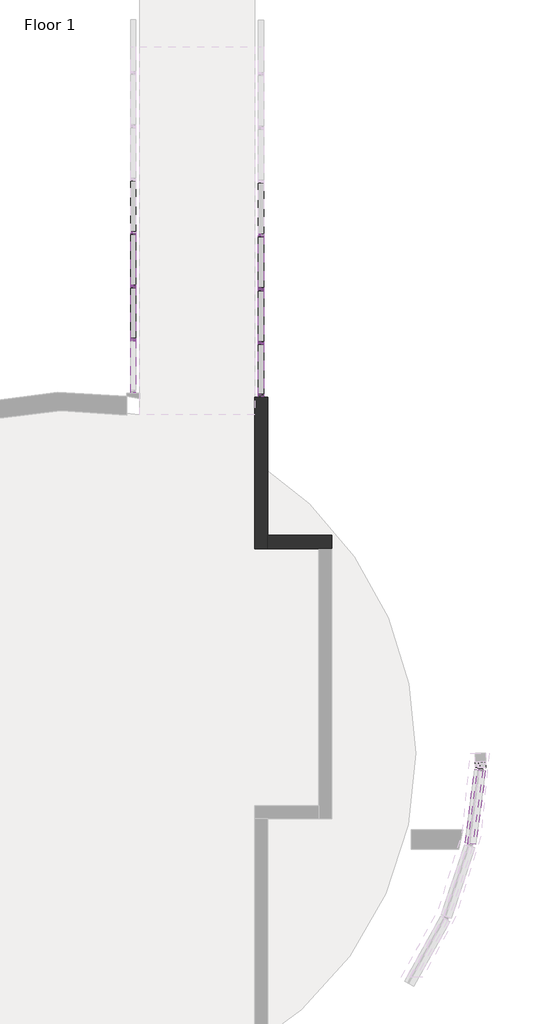
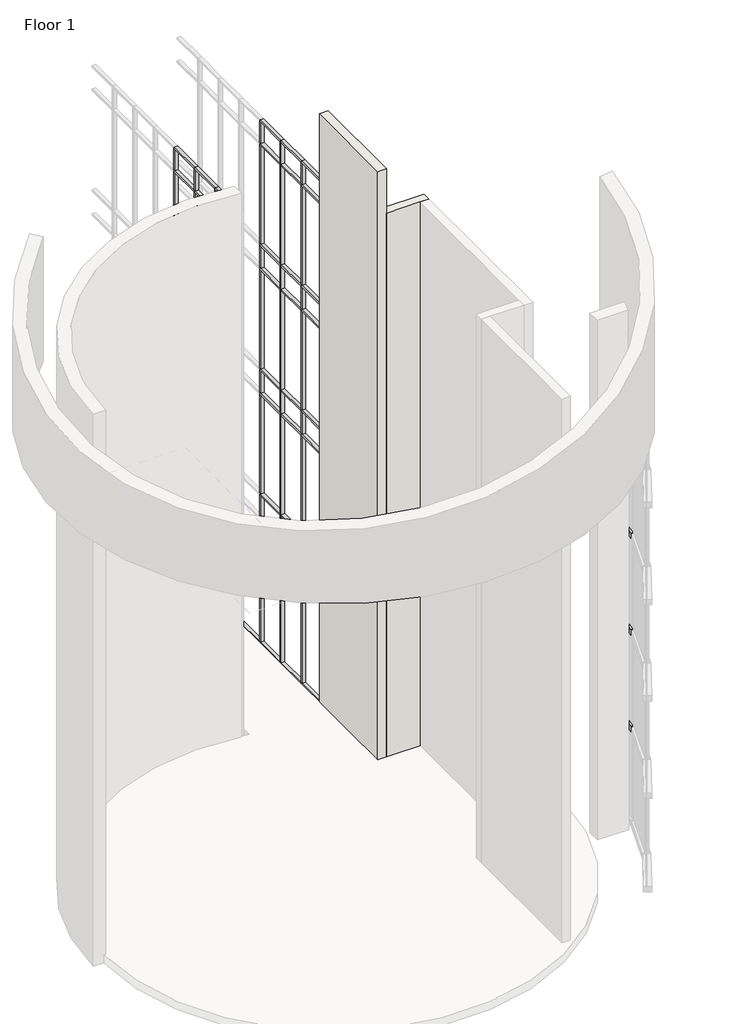
# One storey, part 7 of 11: 111 members, 2 walls.
"""IFC4 building model written with IfcOpenShell, lengths in millimetres."""

import ifcopenshell
import ifcopenshell.guid

model = None  # the IFC model being written
_history = None  # IfcOwnerHistory: only IFC2X3 demands one
_inside = {}  # id of a spatial element -> (the spatial element, [elements in it])
_under = {}  # id of a project, library or spatial element -> (it, [spatial elements below it])
_declared = {}  # id of a project -> (the project, [libraries it declares])
_typed = {}  # id of a type object -> (the type object, [elements of that type])
_made_of = {}  # id of a material, layer set ... -> (it, [elements and type objects made of it])


def new_model(schema):
    """Start an empty IFC model of exactly this schema.

    Asked for "IFC4X3", IfcOpenShell would pick the latest addendum, in which some entities
    have other attributes; the version numbers below select the first issue.
    IFC2X3 requires an IfcOwnerHistory on every rooted entity: one is made here for all.
    """
    global model, _history
    if schema == "IFC4X3":
        model = ifcopenshell.file(schema_version=(4, 3, 0, 0))
    else:
        model = ifcopenshell.file(schema=schema)
    _inside.clear()
    _under.clear()
    _declared.clear()
    _typed.clear()
    _made_of.clear()
    _history = None
    if model.schema == "IFC2X3":
        org = make("IfcOrganization", Name="unknown")
        user = make(
            "IfcPersonAndOrganization",
            ThePerson=make("IfcPerson", FamilyName="unknown"),
            TheOrganization=org,
        )
        app = make(
            "IfcApplication",
            ApplicationDeveloper=org,
            Version="unknown",
            ApplicationFullName="unknown",
            ApplicationIdentifier="unknown",
        )
        _history = make(
            "IfcOwnerHistory",
            OwningUser=user,
            OwningApplication=app,
            ChangeAction="ADDED",
            CreationDate=0,
        )
    return model


def make(cls, **values):
    """One entity of the class cls with the attributes given. An attribute that is None is left unset."""
    return model.create_entity(
        cls, **{name: value for name, value in values.items() if value is not None}
    )


def rooted(cls, **values):
    """An entity with a GlobalId (a new one), such as an element, a storey or a relation."""
    return make(cls, GlobalId=ifcopenshell.guid.new(), OwnerHistory=_history, **values)


def si_unit(unit_type, name, prefix=None):
    """IfcSIUnit, for example si_unit("LENGTHUNIT", "METRE", prefix="MILLI")."""
    return make("IfcSIUnit", UnitType=unit_type, Prefix=prefix, Name=name)


def assignment(units):
    """IfcUnitAssignment: the units of a project."""
    return None if units is None else make("IfcUnitAssignment", Units=units)


def point(xyz):
    """IfcCartesianPoint."""
    return None if xyz is None else make("IfcCartesianPoint", Coordinates=xyz)


def direction(xyz):
    """IfcDirection."""
    return None if xyz is None else make("IfcDirection", DirectionRatios=xyz)


def frame(location, z_axis=None, x_axis=None):
    """IfcAxis2Placement3D, a coordinate frame: its origin and axes. An axis left out is left unset."""
    return make(
        "IfcAxis2Placement3D",
        Location=point(location),
        Axis=direction(z_axis),
        RefDirection=direction(x_axis),
    )


def origin():
    """The frame at (0, 0, 0) with its axes left unset."""
    return frame((0.0, 0.0, 0.0))


def place(relative_to, where):
    """IfcLocalPlacement: puts the frame where relative to a parent placement (None: the world)."""
    return make(
        "IfcLocalPlacement", PlacementRelTo=relative_to, RelativePlacement=where
    )


def context(
    kind, dimensions, precision=None, world=None, true_north=None, identifier=None
):
    """IfcGeometricRepresentationContext, for example the 3D "Model" context."""
    return make(
        "IfcGeometricRepresentationContext",
        ContextIdentifier=identifier,
        ContextType=kind,
        CoordinateSpaceDimension=dimensions,
        Precision=precision,
        WorldCoordinateSystem=world,
        TrueNorth=true_north,
    )


def project(units=None, contexts=None):
    """IfcProject with its units and contexts."""
    return rooted(
        "IfcProject",
        Name="project",
        RepresentationContexts=contexts,
        UnitsInContext=assignment(units),
    )


def spatial(cls, under=None, at=None, **own):
    """A site, building, storey or space (cls), placed at a placement, below another one or the project."""
    s = rooted(cls, ObjectPlacement=at, **own)
    if under is not None:
        _under.setdefault(under.id(), (under, []))[1].append(s)
    return s


def polyline(points):
    """IfcPolyline through the points."""
    return make("IfcPolyline", Points=[point(p) for p in points])


def outline(outer, holes=None, kind="AREA"):
    """IfcArbitraryClosedProfileDef: a profile drawn as a closed curve; with holes, ...WithVoids."""
    if holes is None:
        return make("IfcArbitraryClosedProfileDef", ProfileType=kind, OuterCurve=outer)
    return make(
        "IfcArbitraryProfileDefWithVoids",
        ProfileType=kind,
        OuterCurve=outer,
        InnerCurves=holes,
    )


def extrude(swept, where, along, depth):
    """IfcExtrudedAreaSolid: the profile swept, set in the frame where, extruded along a direction by depth."""
    return make(
        "IfcExtrudedAreaSolid",
        SweptArea=swept,
        Position=where,
        ExtrudedDirection=direction(along),
        Depth=depth,
    )


def faces_of(points, faces, orient=None, outer=None):
    """IfcFace entities. A face is a list of loops; a loop is a list of indices into points, from 0.

    orient and outer hold one flag for each loop. By default every Orientation is true, the
    first loop of a face is its IfcFaceOuterBound and the others are IfcFaceBound.
    """
    made = []
    for i, loops in enumerate(faces):
        bounds = []
        for j, loop in enumerate(loops):
            is_outer = j == 0 if outer is None else outer[i][j]
            bounds.append(
                make(
                    "IfcFaceOuterBound" if is_outer else "IfcFaceBound",
                    Bound=make("IfcPolyLoop", Polygon=[points[k] for k in loop]),
                    Orientation=True if orient is None else orient[i][j],
                )
            )
        made.append(make("IfcFace", Bounds=bounds))
    return made


def faceted_brep(points, faces, orient=None, outer=None, voids=None):
    """IfcFacetedBrep: a solid bounded by flat faces; with voids (closed shells), ...WithVoids."""
    shared = [point(p) for p in points]
    hull = make("IfcClosedShell", CfsFaces=faces_of(shared, faces, orient, outer))
    if voids is None:
        return make("IfcFacetedBrep", Outer=hull)
    return make(
        "IfcFacetedBrepWithVoids",
        Outer=hull,
        Voids=[
            make(cls, CfsFaces=faces_of(shared, fs, o, b)) for cls, fs, o, b in voids
        ],
    )


def shape(context_of_items, identifier, shape_type, items):
    """IfcShapeRepresentation: the items that make up one representation, for example the "Body"."""
    return make(
        "IfcShapeRepresentation",
        ContextOfItems=context_of_items,
        RepresentationIdentifier=identifier,
        RepresentationType=shape_type,
        Items=items,
    )


def source(mapping_origin, context_of_items, identifier, shape_type, items):
    """IfcRepresentationMap: a shape defined once, which mapped items show again and again."""
    return make(
        "IfcRepresentationMap",
        MappingOrigin=mapping_origin,
        MappedRepresentation=shape(context_of_items, identifier, shape_type, items),
    )


def transform(
    local_origin,
    x_axis=None,
    y_axis=None,
    z_axis=None,
    scale=None,
    scale2=None,
    scale3=None,
    uniform=True,
):
    """IfcCartesianTransformationOperator3D, or its non-uniform kind. x_axis, y_axis, z_axis: its Axis1, 2, 3."""
    if uniform:
        return make(
            "IfcCartesianTransformationOperator3D",
            Axis1=direction(x_axis),
            Axis2=direction(y_axis),
            LocalOrigin=point(local_origin),
            Scale=scale,
            Axis3=direction(z_axis),
        )
    return make(
        "IfcCartesianTransformationOperator3DnonUniform",
        Axis1=direction(x_axis),
        Axis2=direction(y_axis),
        LocalOrigin=point(local_origin),
        Scale=scale,
        Axis3=direction(z_axis),
        Scale2=scale2,
        Scale3=scale3,
    )


def mapped(mapping_source, mapping_target):
    """IfcMappedItem: shows the shape of a source again, moved by a transform."""
    return make(
        "IfcMappedItem", MappingSource=mapping_source, MappingTarget=mapping_target
    )


def made_of(thing, what):
    """Note that an element or type object is made of a material, layer set ...; save() writes the relation."""
    if what is not None:
        _made_of.setdefault(what.id(), (what, []))[1].append(thing)
    return thing


def element(
    cls,
    number,
    at=None,
    inside=None,
    cuts=None,
    type_object=None,
    material=None,
    context=None,
    identifier="Body",
    shape_type=None,
    held_by="IfcProductDefinitionShape",
    body=None,
    shapes=None,
    **own,
):
    """One element of the class cls, such as IfcWall. Its Tag is "e" and its number.

    at: its placement. inside: the storey or other place that contains it. cuts: it is an
    opening in that element (IfcRelVoidsElement). A single representation is given by context,
    identifier, shape_type and body (its items); several are given by shapes. held_by: the class
    of the entity that holds the representations. save() writes the other relations.
    """
    e = rooted(cls, Tag="e%d" % number, ObjectPlacement=at, **own)
    if body is not None:
        shapes = [shape(context, identifier, shape_type, body)]
    if shapes is not None:
        e.Representation = make(held_by, Representations=shapes)
    if inside is not None:
        _inside.setdefault(inside.id(), (inside, []))[1].append(e)
    if cuts is not None:
        rooted(
            "IfcRelVoidsElement", RelatingBuildingElement=cuts, RelatedOpeningElement=e
        )
    if type_object is not None:
        _typed.setdefault(type_object.id(), (type_object, []))[1].append(e)
    return made_of(e, material)


def aggregate(whole, parts):
    """IfcRelAggregates: a whole, such as a stair, and the parts it consists of."""
    return rooted("IfcRelAggregates", RelatingObject=whole, RelatedObjects=parts)


def save(model, path):
    """Write the relations noted so far, then the file.

    IfcRelAggregates (storeys below a building ...), IfcRelContainedInSpatialStructure (elements
    in a storey), IfcRelDefinesByType, IfcRelAssociatesMaterial and IfcRelDeclares: one each for
    every whole, place, type object, material and project.
    """
    for whole, parts in _under.values():
        aggregate(whole, parts)
    for where, things in _inside.values():
        rooted(
            "IfcRelContainedInSpatialStructure",
            RelatedElements=things,
            RelatingStructure=where,
        )
    for kind, things in _typed.values():
        rooted("IfcRelDefinesByType", RelatedObjects=things, RelatingType=kind)
    for what, things in _made_of.values():
        rooted("IfcRelAssociatesMaterial", RelatedObjects=things, RelatingMaterial=what)
    for by, libraries in _declared.values():
        rooted("IfcRelDeclares", RelatingContext=by, RelatedDefinitions=libraries)
    model.write(path)


def member_5d07894b(model_context):
    return source(origin(), model_context, "Body", "SweptSolid", [
        extrude(outline(polyline([(31.75, 63.5), (31.75, -63.5), (-31.75, -63.5), (-31.75, 63.5), (31.75, 63.5)])), frame((0.0, 0.0, -4629.15), z_axis=(0.0, 0.0, 1.0), x_axis=(1.0, 0.0, 0.0)), (0.0, 0.0, 1.0), 4629.15),
    ])


def member_c86c7f77(model_context):
    return source(origin(), model_context, "Body", "SweptSolid", [
        extrude(outline(polyline([(31.75, 63.5), (31.75, -63.5), (-31.75, -63.5), (-31.75, 63.5), (31.75, 63.5)])), frame((0.0, 0.0, -1270.9989637), z_axis=(0.0, 0.0, 1.0), x_axis=(1.0, 0.0, 0.0)), (0.0, 0.0, 1.0), 1270.9989637),
    ])


def member_60e3aab2(model_context):
    return source(origin(), model_context, "Body", "SweptSolid", [
        extrude(outline(polyline([(0.0, 63.5), (0.0, -63.5), (-63.5, -63.5), (-63.5, 63.5), (0.0, 63.5)])), frame((0.0, 0.0, -1270.9989637), z_axis=(0.0, 0.0, 1.0), x_axis=(1.0, 0.0, 0.0)), (0.0, 0.0, 1.0), 1270.9989637),
    ])


def member_3ba9e939(model_context):
    return source(origin(), model_context, "Body", "SweptSolid", [
        extrude(outline(polyline([(31.75, 63.5), (31.75, -63.5), (-31.75, -63.5), (-31.75, 63.5), (31.75, 63.5)])), frame((0.0, 0.0, -3746.5), z_axis=(0.0, 0.0, 1.0), x_axis=(1.0, 0.0, 0.0)), (0.0, 0.0, 1.0), 3746.5),
    ])


def member_ad567e07(model_context):
    return source(origin(), model_context, "Body", "SweptSolid", [
        extrude(outline(polyline([(31.75, 63.5), (31.75, -63.5), (-31.75, -63.5), (-31.75, 63.5), (31.75, 63.5)])), frame((0.0, 0.0, -819.15), z_axis=(0.0, 0.0, 1.0), x_axis=(1.0, 0.0, 0.0)), (0.0, 0.0, 1.0), 819.15),
    ])


def member_7db1855a(model_context):
    return source(origin(), model_context, "Body", "SweptSolid", [
        extrude(outline(polyline([(31.75, 63.5), (31.75, -63.5), (-31.75, -63.5), (-31.75, 63.5), (31.75, 63.5)])), frame((0.0, 0.0, -850.9), z_axis=(0.0, 0.0, 1.0), x_axis=(1.0, 0.0, 0.0)), (0.0, 0.0, 1.0), 850.9),
    ])


def member_5783932f(model_context):
    return source(origin(), model_context, "Body", "SweptSolid", [
        extrude(outline(polyline([(0.0, 63.5), (0.0, -63.5), (-63.5, -63.5), (-63.5, 63.5), (0.0, 63.5)])), frame((0.0, 0.0, -1282.7), z_axis=(0.0, 0.0, 1.0), x_axis=(1.0, 0.0, 0.0)), (0.0, 0.0, 1.0), 1282.7),
    ])


def member_98b79ab6(model_context):
    return source(origin(), model_context, "Body", "SweptSolid", [
        extrude(outline(polyline([(31.75, 63.5), (31.75, -63.5), (-31.75, -63.5), (-31.75, 63.5), (31.75, 63.5)])), frame((0.0, 0.0, -1282.7), z_axis=(0.0, 0.0, 1.0), x_axis=(1.0, 0.0, 0.0)), (0.0, 0.0, 1.0), 1282.7),
    ])


def member_810865a4(model_context):
    return source(origin(), model_context, "Body", "SweptSolid", [
        extrude(outline(polyline([(31.75, 63.5), (31.75, -63.5), (-31.75, -63.5), (-31.75, 63.5), (31.75, 63.5)])), frame((0.0, 0.0, -3657.6), z_axis=(0.0, 0.0, 1.0), x_axis=(1.0, 0.0, 0.0)), (0.0, 0.0, 1.0), 3657.6),
    ])


def member_b9454cfc(model_context):
    return source(origin(), model_context, "Body", "SweptSolid", [
        extrude(outline(polyline([(-63.5, 28.7582862), (-60.2336356, -5.8295375), (63.5, 5.8554746), (63.5, -1771.1554746), (-60.2336356, -1759.4704625), (-63.5, -1794.0582862), (-63.5, 28.7582862)])), frame((-63.5, 0.0, 0.0), z_axis=(1.0, 0.0, 0.0), x_axis=(0.0, 1.0, 0.0)), (0.0, 0.0, 1.0), 63.5),
    ])


def member_c17f1be2(model_context):
    return source(origin(), model_context, "Body", "SweptSolid", [
        extrude(outline(polyline([(0.0, 63.5), (0.0, -63.5), (-63.5, -63.5), (-63.5, 63.5), (0.0, 63.5)])), frame((0.0, 0.0, -819.15), z_axis=(0.0, 0.0, 1.0), x_axis=(1.0, 0.0, 0.0)), (0.0, 0.0, 1.0), 819.15),
    ])


def member_d2e7e466(model_context):
    return source(origin(), model_context, "Body", "SweptSolid", [
        extrude(outline(polyline([(0.0, 63.5), (0.0, -63.5), (-63.5, -63.5), (-63.5, 63.5), (0.0, 63.5)])), frame((0.0, 0.0, -850.9), z_axis=(0.0, 0.0, 1.0), x_axis=(1.0, 0.0, 0.0)), (0.0, 0.0, 1.0), 850.9),
    ])


def member_bbf28ac8(model_context):
    return source(origin(), model_context, "Body", "SweptSolid", [
        extrude(outline(polyline([(0.0, 63.5), (0.0, -63.5), (-63.5, -63.5), (-63.5, 63.5), (0.0, 63.5)])), frame((0.0, 0.0, -3746.5), z_axis=(0.0, 0.0, 1.0), x_axis=(1.0, 0.0, 0.0)), (0.0, 0.0, 1.0), 3746.5),
    ])


def member_5c8c9790(model_context):
    return source(origin(), model_context, "Body", "SweptSolid", [
        extrude(outline(polyline([(0.0, 63.5), (0.0, -63.5), (-63.5, -63.5), (-63.5, 63.5), (0.0, 63.5)])), frame((0.0, 0.0, -4629.15), z_axis=(0.0, 0.0, 1.0), x_axis=(1.0, 0.0, 0.0)), (0.0, 0.0, 1.0), 4629.15),
    ])


def member_93925f5f(model_context):
    return source(origin(), model_context, "Body", "SweptSolid", [
        extrude(outline(polyline([(0.0, 127.0), (0.0, -127.0), (-203.2, -127.0), (-203.2, 127.0), (0.0, 127.0)])), frame((0.0, 0.0, -139.2998379), z_axis=(0.0, 0.0, 1.0), x_axis=(1.0, 0.0, 0.0)), (0.0, 0.0, 1.0), 139.2998379),
    ])


def member_707c4438(model_context):
    return source(origin(), model_context, "Body", "SweptSolid", [
        extrude(outline(polyline([(101.6, 127.0), (101.6, -127.0), (-101.6, -127.0), (-101.6, 127.0), (101.6, 127.0)])), frame((0.0, 0.0, -1765.3), z_axis=(0.0, 0.0, 1.0), x_axis=(1.0, 0.0, 0.0)), (0.0, 0.0, 1.0), 1765.3),
    ])


model = new_model("IFC4")

# Units and contexts
model_context = context("Model", 3, world=origin())
ifc_project = project(units=[si_unit("LENGTHUNIT", "METRE", prefix="MILLI")], contexts=[model_context])

# Site, building, storey
site = spatial("IfcSite", under=ifc_project)
building = spatial("IfcBuilding", under=site)
storey = spatial("IfcBuildingStorey", under=building, Name="Floor 1", Elevation=0.0)

# Members
placement = place(None, origin())
member_shape = member_5d07894b(model_context)
element("IfcMember", 1, ObjectType="Rectangular Mullion1 : 2.5\" x 5\" rectangular", at=placement, inside=storey, context=model_context, shape_type="MappedRepresentation", body=[
    mapped(member_shape, transform((10878.8276119, 30390.311889, -88.9), x_axis=(0.0, 1.0, 0.0), y_axis=(1.0, 0.0, 0.0), z_axis=(0.0, 0.0, -1.0))),
])
element("IfcMember", 2, ObjectType="Rectangular Mullion1 : 2.5\" x 5\" rectangular", at=placement, inside=storey, context=model_context, shape_type="MappedRepresentation", body=[
    mapped(member_shape, transform((10878.8276119, 29107.611889, -88.9), x_axis=(0.0, 1.0, 0.0), y_axis=(1.0, 0.0, 0.0), z_axis=(0.0, 0.0, -1.0))),
])
element("IfcMember", 3, ObjectType="Rectangular Mullion1 : 2.5\" x 5\" rectangular", at=placement, inside=storey, context=model_context, shape_type="MappedRepresentation", body=[
    mapped(member_shape, transform((10878.8276119, 31673.011889, -88.9), x_axis=(0.0, 1.0, 0.0), y_axis=(1.0, 0.0, 0.0), z_axis=(0.0, 0.0, -1.0))),
])
element("IfcMember", 4, ObjectType="Rectangular Mullion1 : 2.5\" x 5\" rectangular", at=placement, inside=storey, context=model_context, shape_type="MappedRepresentation", body=[
    mapped(member_shape, transform((7830.8276119, 30460.5181066, -88.9), x_axis=(0.0, 1.0, 0.0), y_axis=(1.0, 0.0, 0.0), z_axis=(0.0, 0.0, -1.0))),
])
element("IfcMember", 5, ObjectType="Rectangular Mullion1 : 2.5\" x 5\" rectangular", at=placement, inside=storey, context=model_context, shape_type="MappedRepresentation", body=[
    mapped(member_shape, transform((7830.8276119, 31731.5170704, -88.9), x_axis=(0.0, 1.0, 0.0), y_axis=(1.0, 0.0, 0.0), z_axis=(0.0, 0.0, -1.0))),
])
member_2_shape = member_c86c7f77(model_context)
element("IfcMember", 6, ObjectType="Rectangular Mullion1 : 2.5\" x 5\" rectangular", at=placement, inside=storey, context=model_context, shape_type="MappedRepresentation", body=[
    mapped(member_2_shape, transform((7830.8276119, 31731.5170704, 5486.4), x_axis=(0.0, 0.0, 1.0), y_axis=(1.0, 0.0, 0.0), z_axis=(0.0, 1.0, 0.0))),
])
element("IfcMember", 7, ObjectType="Rectangular Mullion1 : 2.5\" x 5\" rectangular", at=placement, inside=storey, context=model_context, shape_type="MappedRepresentation", body=[
    mapped(member_2_shape, transform((7830.8276119, 30460.5181066, 5486.4), x_axis=(0.0, 0.0, 1.0), y_axis=(1.0, 0.0, 0.0), z_axis=(0.0, 1.0, 0.0))),
])
element("IfcMember", 8, ObjectType="Rectangular Mullion1 : 2.5\" x 5\" rectangular", at=placement, inside=storey, context=model_context, shape_type="MappedRepresentation", body=[
    mapped(member_2_shape, transform((7830.8276119, 31731.5170704, 10210.8), x_axis=(0.0, 0.0, 1.0), y_axis=(1.0, 0.0, 0.0), z_axis=(0.0, 1.0, 0.0))),
])
element("IfcMember", 9, ObjectType="Rectangular Mullion1 : 2.5\" x 5\" rectangular", at=placement, inside=storey, context=model_context, shape_type="MappedRepresentation", body=[
    mapped(member_2_shape, transform((7830.8276119, 30460.5181066, 10210.8), x_axis=(0.0, 0.0, 1.0), y_axis=(1.0, 0.0, 0.0), z_axis=(0.0, 1.0, 0.0))),
])
element("IfcMember", 10, ObjectType="Rectangular Mullion1 : 2.5\" x 5\" rectangular", at=placement, inside=storey, context=model_context, shape_type="MappedRepresentation", body=[
    mapped(member_2_shape, transform((7830.8276119, 31731.5170704, 14935.2), x_axis=(0.0, 0.0, 1.0), y_axis=(1.0, 0.0, 0.0), z_axis=(0.0, 1.0, 0.0))),
])
element("IfcMember", 11, ObjectType="Rectangular Mullion1 : 2.5\" x 5\" rectangular", at=placement, inside=storey, context=model_context, shape_type="MappedRepresentation", body=[
    mapped(member_2_shape, transform((7830.8276119, 30460.5181066, 14935.2), x_axis=(0.0, 0.0, 1.0), y_axis=(1.0, 0.0, 0.0), z_axis=(0.0, 1.0, 0.0))),
])
element("IfcMember", 12, ObjectType="Rectangular Mullion1 : 2.5\" x 5\" rectangular", at=placement, inside=storey, context=model_context, shape_type="MappedRepresentation", body=[
    mapped(member_2_shape, transform((7830.8276119, 31731.5170704, 18745.2), x_axis=(0.0, 0.0, 1.0), y_axis=(1.0, 0.0, 0.0), z_axis=(0.0, 1.0, 0.0))),
])
element("IfcMember", 13, ObjectType="Rectangular Mullion1 : 2.5\" x 5\" rectangular", at=placement, inside=storey, context=model_context, shape_type="MappedRepresentation", body=[
    mapped(member_2_shape, transform((7830.8276119, 30460.5181066, 18745.2), x_axis=(0.0, 0.0, 1.0), y_axis=(1.0, 0.0, 0.0), z_axis=(0.0, 1.0, 0.0))),
])
element("IfcMember", 14, ObjectType="Rectangular Mullion1 : 2.5\" x 5\" rectangular", at=placement, inside=storey, context=model_context, shape_type="MappedRepresentation", body=[
    mapped(member_2_shape, transform((7830.8276119, 31731.5170704, 14020.8), x_axis=(0.0, 0.0, 1.0), y_axis=(1.0, 0.0, 0.0), z_axis=(0.0, 1.0, 0.0))),
])
element("IfcMember", 15, ObjectType="Rectangular Mullion1 : 2.5\" x 5\" rectangular", at=placement, inside=storey, context=model_context, shape_type="MappedRepresentation", body=[
    mapped(member_2_shape, transform((7830.8276119, 30460.5181066, 14020.8), x_axis=(0.0, 0.0, 1.0), y_axis=(1.0, 0.0, 0.0), z_axis=(0.0, 1.0, 0.0))),
])
element("IfcMember", 16, ObjectType="Rectangular Mullion1 : 2.5\" x 5\" rectangular", at=placement, inside=storey, context=model_context, shape_type="MappedRepresentation", body=[
    mapped(member_2_shape, transform((7830.8276119, 31731.5170704, 9296.4), x_axis=(0.0, 0.0, 1.0), y_axis=(1.0, 0.0, 0.0), z_axis=(0.0, 1.0, 0.0))),
])
element("IfcMember", 17, ObjectType="Rectangular Mullion1 : 2.5\" x 5\" rectangular", at=placement, inside=storey, context=model_context, shape_type="MappedRepresentation", body=[
    mapped(member_2_shape, transform((7830.8276119, 30460.5181066, 9296.4), x_axis=(0.0, 0.0, 1.0), y_axis=(1.0, 0.0, 0.0), z_axis=(0.0, 1.0, 0.0))),
])
element("IfcMember", 18, ObjectType="Rectangular Mullion1 : 2.5\" x 5\" rectangular", at=placement, inside=storey, context=model_context, shape_type="MappedRepresentation", body=[
    mapped(member_2_shape, transform((7830.8276119, 31731.5170704, 4572.0), x_axis=(0.0, 0.0, 1.0), y_axis=(1.0, 0.0, 0.0), z_axis=(0.0, 1.0, 0.0))),
])
element("IfcMember", 19, ObjectType="Rectangular Mullion1 : 2.5\" x 5\" rectangular", at=placement, inside=storey, context=model_context, shape_type="MappedRepresentation", body=[
    mapped(member_2_shape, transform((7830.8276119, 30460.5181066, 4572.0), x_axis=(0.0, 0.0, 1.0), y_axis=(1.0, 0.0, 0.0), z_axis=(0.0, 1.0, 0.0))),
])
member_3_shape = member_60e3aab2(model_context)
element("IfcMember", 20, ObjectType="Rectangular Mullion1 : 2.5\" x 5\" rectangular", at=placement, inside=storey, context=model_context, shape_type="MappedRepresentation", body=[
    mapped(member_3_shape, transform((7830.8276119, 30460.5181066, -152.4), x_axis=(0.0, 0.0, -1.0), y_axis=(1.0, 0.0, 0.0), z_axis=(0.0, -1.0, 0.0))),
])
element("IfcMember", 21, ObjectType="Rectangular Mullion1 : 2.5\" x 5\" rectangular", at=placement, inside=storey, context=model_context, shape_type="MappedRepresentation", body=[
    mapped(member_3_shape, transform((7830.8276119, 31731.5170704, -152.4), x_axis=(0.0, 0.0, -1.0), y_axis=(1.0, 0.0, 0.0), z_axis=(0.0, -1.0, 0.0))),
])
element("IfcMember", 22, ObjectType="Rectangular Mullion1 : 2.5\" x 5\" rectangular", at=placement, inside=storey, context=model_context, shape_type="MappedRepresentation", body=[
    mapped(member_3_shape, transform((7830.8276119, 29189.5191429, -152.4), x_axis=(0.0, 0.0, -1.0), y_axis=(1.0, 0.0, 0.0), z_axis=(0.0, -1.0, 0.0))),
])
element("IfcMember", 23, ObjectType="Rectangular Mullion1 : 2.5\" x 5\" rectangular", at=placement, inside=storey, context=model_context, shape_type="MappedRepresentation", body=[
    mapped(member_3_shape, transform((7830.8276119, 30460.5181066, 19659.6), x_axis=(0.0, 0.0, 1.0), y_axis=(1.0, 0.0, 0.0), z_axis=(0.0, 1.0, 0.0))),
])
element("IfcMember", 24, ObjectType="Rectangular Mullion1 : 2.5\" x 5\" rectangular", at=placement, inside=storey, context=model_context, shape_type="MappedRepresentation", body=[
    mapped(member_3_shape, transform((7830.8276119, 31731.5170704, 19659.6), x_axis=(0.0, 0.0, 1.0), y_axis=(1.0, 0.0, 0.0), z_axis=(0.0, 1.0, 0.0))),
])
element("IfcMember", 25, ObjectType="Rectangular Mullion1 : 2.5\" x 5\" rectangular", at=placement, inside=storey, context=model_context, shape_type="MappedRepresentation", body=[
    mapped(member_3_shape, transform((7830.8276119, 29189.5191429, 19659.6), x_axis=(0.0, 0.0, 1.0), y_axis=(1.0, 0.0, 0.0), z_axis=(0.0, 1.0, 0.0))),
])
member_4_shape = member_3ba9e939(model_context)
element("IfcMember", 26, ObjectType="Rectangular Mullion1 : 2.5\" x 5\" rectangular", at=placement, inside=storey, context=model_context, shape_type="MappedRepresentation", body=[
    mapped(member_4_shape, transform((10878.8276119, 30390.311889, 14966.95), x_axis=(0.0, 1.0, 0.0), y_axis=(1.0, 0.0, 0.0), z_axis=(0.0, 0.0, -1.0))),
])
element("IfcMember", 27, ObjectType="Rectangular Mullion1 : 2.5\" x 5\" rectangular", at=placement, inside=storey, context=model_context, shape_type="MappedRepresentation", body=[
    mapped(member_4_shape, transform((10878.8276119, 30390.311889, 10242.55), x_axis=(0.0, 1.0, 0.0), y_axis=(1.0, 0.0, 0.0), z_axis=(0.0, 0.0, -1.0))),
])
element("IfcMember", 28, ObjectType="Rectangular Mullion1 : 2.5\" x 5\" rectangular", at=placement, inside=storey, context=model_context, shape_type="MappedRepresentation", body=[
    mapped(member_4_shape, transform((10878.8276119, 30390.311889, 5518.15), x_axis=(0.0, 1.0, 0.0), y_axis=(1.0, 0.0, 0.0), z_axis=(0.0, 0.0, -1.0))),
])
element("IfcMember", 29, ObjectType="Rectangular Mullion1 : 2.5\" x 5\" rectangular", at=placement, inside=storey, context=model_context, shape_type="MappedRepresentation", body=[
    mapped(member_4_shape, transform((10878.8276119, 29107.611889, 14966.95), x_axis=(0.0, 1.0, 0.0), y_axis=(1.0, 0.0, 0.0), z_axis=(0.0, 0.0, -1.0))),
])
element("IfcMember", 30, ObjectType="Rectangular Mullion1 : 2.5\" x 5\" rectangular", at=placement, inside=storey, context=model_context, shape_type="MappedRepresentation", body=[
    mapped(member_4_shape, transform((10878.8276119, 29107.611889, 10242.55), x_axis=(0.0, 1.0, 0.0), y_axis=(1.0, 0.0, 0.0), z_axis=(0.0, 0.0, -1.0))),
])
element("IfcMember", 31, ObjectType="Rectangular Mullion1 : 2.5\" x 5\" rectangular", at=placement, inside=storey, context=model_context, shape_type="MappedRepresentation", body=[
    mapped(member_4_shape, transform((10878.8276119, 29107.611889, 5518.15), x_axis=(0.0, 1.0, 0.0), y_axis=(1.0, 0.0, 0.0), z_axis=(0.0, 0.0, -1.0))),
])
element("IfcMember", 32, ObjectType="Rectangular Mullion1 : 2.5\" x 5\" rectangular", at=placement, inside=storey, context=model_context, shape_type="MappedRepresentation", body=[
    mapped(member_4_shape, transform((10878.8276119, 31673.011889, 14966.95), x_axis=(0.0, 1.0, 0.0), y_axis=(1.0, 0.0, 0.0), z_axis=(0.0, 0.0, -1.0))),
])
element("IfcMember", 33, ObjectType="Rectangular Mullion1 : 2.5\" x 5\" rectangular", at=placement, inside=storey, context=model_context, shape_type="MappedRepresentation", body=[
    mapped(member_4_shape, transform((10878.8276119, 31673.011889, 10242.55), x_axis=(0.0, 1.0, 0.0), y_axis=(1.0, 0.0, 0.0), z_axis=(0.0, 0.0, -1.0))),
])
element("IfcMember", 34, ObjectType="Rectangular Mullion1 : 2.5\" x 5\" rectangular", at=placement, inside=storey, context=model_context, shape_type="MappedRepresentation", body=[
    mapped(member_4_shape, transform((10878.8276119, 31673.011889, 5518.15), x_axis=(0.0, 1.0, 0.0), y_axis=(1.0, 0.0, 0.0), z_axis=(0.0, 0.0, -1.0))),
])
element("IfcMember", 35, ObjectType="Rectangular Mullion1 : 2.5\" x 5\" rectangular", at=placement, inside=storey, context=model_context, shape_type="MappedRepresentation", body=[
    mapped(member_4_shape, transform((7830.8276119, 30460.5181066, 5518.15), x_axis=(0.0, 1.0, 0.0), y_axis=(1.0, 0.0, 0.0), z_axis=(0.0, 0.0, -1.0))),
])
element("IfcMember", 36, ObjectType="Rectangular Mullion1 : 2.5\" x 5\" rectangular", at=placement, inside=storey, context=model_context, shape_type="MappedRepresentation", body=[
    mapped(member_4_shape, transform((7830.8276119, 30460.5181066, 10242.55), x_axis=(0.0, 1.0, 0.0), y_axis=(1.0, 0.0, 0.0), z_axis=(0.0, 0.0, -1.0))),
])
element("IfcMember", 37, ObjectType="Rectangular Mullion1 : 2.5\" x 5\" rectangular", at=placement, inside=storey, context=model_context, shape_type="MappedRepresentation", body=[
    mapped(member_4_shape, transform((7830.8276119, 30460.5181066, 14966.95), x_axis=(0.0, 1.0, 0.0), y_axis=(1.0, 0.0, 0.0), z_axis=(0.0, 0.0, -1.0))),
])
element("IfcMember", 38, ObjectType="Rectangular Mullion1 : 2.5\" x 5\" rectangular", at=placement, inside=storey, context=model_context, shape_type="MappedRepresentation", body=[
    mapped(member_4_shape, transform((7830.8276119, 31731.5170704, 5518.15), x_axis=(0.0, 1.0, 0.0), y_axis=(1.0, 0.0, 0.0), z_axis=(0.0, 0.0, -1.0))),
])
element("IfcMember", 39, ObjectType="Rectangular Mullion1 : 2.5\" x 5\" rectangular", at=placement, inside=storey, context=model_context, shape_type="MappedRepresentation", body=[
    mapped(member_4_shape, transform((7830.8276119, 31731.5170704, 10242.55), x_axis=(0.0, 1.0, 0.0), y_axis=(1.0, 0.0, 0.0), z_axis=(0.0, 0.0, -1.0))),
])
element("IfcMember", 40, ObjectType="Rectangular Mullion1 : 2.5\" x 5\" rectangular", at=placement, inside=storey, context=model_context, shape_type="MappedRepresentation", body=[
    mapped(member_4_shape, transform((7830.8276119, 31731.5170704, 14966.95), x_axis=(0.0, 1.0, 0.0), y_axis=(1.0, 0.0, 0.0), z_axis=(0.0, 0.0, -1.0))),
])
element("IfcMember", 41, ObjectType="Rectangular Mullion1 : 2.5\" x 5\" rectangular", at=placement, inside=storey, context=model_context, shape_type="MappedRepresentation", body=[
    mapped(member_4_shape, transform((7830.8276119, 29189.5191429, 5518.15), x_axis=(0.0, 1.0, 0.0), y_axis=(1.0, 0.0, 0.0), z_axis=(0.0, 0.0, -1.0))),
])
element("IfcMember", 42, ObjectType="Rectangular Mullion1 : 2.5\" x 5\" rectangular", at=placement, inside=storey, context=model_context, shape_type="MappedRepresentation", body=[
    mapped(member_4_shape, transform((7830.8276119, 29189.5191429, 10242.55), x_axis=(0.0, 1.0, 0.0), y_axis=(1.0, 0.0, 0.0), z_axis=(0.0, 0.0, -1.0))),
])
element("IfcMember", 43, ObjectType="Rectangular Mullion1 : 2.5\" x 5\" rectangular", at=placement, inside=storey, context=model_context, shape_type="MappedRepresentation", body=[
    mapped(member_4_shape, transform((7830.8276119, 29189.5191429, 14966.95), x_axis=(0.0, 1.0, 0.0), y_axis=(1.0, 0.0, 0.0), z_axis=(0.0, 0.0, -1.0))),
])
member_5_shape = member_ad567e07(model_context)
element("IfcMember", 44, ObjectType="Rectangular Mullion1 : 2.5\" x 5\" rectangular", at=placement, inside=storey, context=model_context, shape_type="MappedRepresentation", body=[
    mapped(member_5_shape, transform((10878.8276119, 30390.311889, 18776.95), x_axis=(0.0, 1.0, 0.0), y_axis=(1.0, 0.0, 0.0), z_axis=(0.0, 0.0, -1.0))),
])
element("IfcMember", 45, ObjectType="Rectangular Mullion1 : 2.5\" x 5\" rectangular", at=placement, inside=storey, context=model_context, shape_type="MappedRepresentation", body=[
    mapped(member_5_shape, transform((10878.8276119, 29107.611889, 18776.95), x_axis=(0.0, 1.0, 0.0), y_axis=(1.0, 0.0, 0.0), z_axis=(0.0, 0.0, -1.0))),
])
element("IfcMember", 46, ObjectType="Rectangular Mullion1 : 2.5\" x 5\" rectangular", at=placement, inside=storey, context=model_context, shape_type="MappedRepresentation", body=[
    mapped(member_5_shape, transform((10878.8276119, 31673.011889, 18776.95), x_axis=(0.0, 1.0, 0.0), y_axis=(1.0, 0.0, 0.0), z_axis=(0.0, 0.0, -1.0))),
])
element("IfcMember", 47, ObjectType="Rectangular Mullion1 : 2.5\" x 5\" rectangular", at=placement, inside=storey, context=model_context, shape_type="MappedRepresentation", body=[
    mapped(member_5_shape, transform((7830.8276119, 30460.5181066, 18776.95), x_axis=(0.0, 1.0, 0.0), y_axis=(1.0, 0.0, 0.0), z_axis=(0.0, 0.0, -1.0))),
])
element("IfcMember", 48, ObjectType="Rectangular Mullion1 : 2.5\" x 5\" rectangular", at=placement, inside=storey, context=model_context, shape_type="MappedRepresentation", body=[
    mapped(member_5_shape, transform((7830.8276119, 31731.5170704, 18776.95), x_axis=(0.0, 1.0, 0.0), y_axis=(1.0, 0.0, 0.0), z_axis=(0.0, 0.0, -1.0))),
])
element("IfcMember", 49, ObjectType="Rectangular Mullion1 : 2.5\" x 5\" rectangular", at=placement, inside=storey, context=model_context, shape_type="MappedRepresentation", body=[
    mapped(member_5_shape, transform((7830.8276119, 29189.5191429, 18776.95), x_axis=(0.0, 1.0, 0.0), y_axis=(1.0, 0.0, 0.0), z_axis=(0.0, 0.0, -1.0))),
])
member_6_shape = member_7db1855a(model_context)
element("IfcMember", 50, ObjectType="Rectangular Mullion1 : 2.5\" x 5\" rectangular", at=placement, inside=storey, context=model_context, shape_type="MappedRepresentation", body=[
    mapped(member_6_shape, transform((10878.8276119, 30390.311889, 9328.15), x_axis=(0.0, 1.0, 0.0), y_axis=(1.0, 0.0, 0.0), z_axis=(0.0, 0.0, -1.0))),
])
element("IfcMember", 51, ObjectType="Rectangular Mullion1 : 2.5\" x 5\" rectangular", at=placement, inside=storey, context=model_context, shape_type="MappedRepresentation", body=[
    mapped(member_6_shape, transform((10878.8276119, 30390.311889, 4603.75), x_axis=(0.0, 1.0, 0.0), y_axis=(1.0, 0.0, 0.0), z_axis=(0.0, 0.0, -1.0))),
])
element("IfcMember", 52, ObjectType="Rectangular Mullion1 : 2.5\" x 5\" rectangular", at=placement, inside=storey, context=model_context, shape_type="MappedRepresentation", body=[
    mapped(member_6_shape, transform((10878.8276119, 30390.311889, 14052.55), x_axis=(0.0, 1.0, 0.0), y_axis=(1.0, 0.0, 0.0), z_axis=(0.0, 0.0, -1.0))),
])
element("IfcMember", 53, ObjectType="Rectangular Mullion1 : 2.5\" x 5\" rectangular", at=placement, inside=storey, context=model_context, shape_type="MappedRepresentation", body=[
    mapped(member_6_shape, transform((10878.8276119, 29107.611889, 9328.15), x_axis=(0.0, 1.0, 0.0), y_axis=(1.0, 0.0, 0.0), z_axis=(0.0, 0.0, -1.0))),
])
element("IfcMember", 54, ObjectType="Rectangular Mullion1 : 2.5\" x 5\" rectangular", at=placement, inside=storey, context=model_context, shape_type="MappedRepresentation", body=[
    mapped(member_6_shape, transform((10878.8276119, 29107.611889, 4603.75), x_axis=(0.0, 1.0, 0.0), y_axis=(1.0, 0.0, 0.0), z_axis=(0.0, 0.0, -1.0))),
])
element("IfcMember", 55, ObjectType="Rectangular Mullion1 : 2.5\" x 5\" rectangular", at=placement, inside=storey, context=model_context, shape_type="MappedRepresentation", body=[
    mapped(member_6_shape, transform((10878.8276119, 29107.611889, 14052.55), x_axis=(0.0, 1.0, 0.0), y_axis=(1.0, 0.0, 0.0), z_axis=(0.0, 0.0, -1.0))),
])
element("IfcMember", 56, ObjectType="Rectangular Mullion1 : 2.5\" x 5\" rectangular", at=placement, inside=storey, context=model_context, shape_type="MappedRepresentation", body=[
    mapped(member_6_shape, transform((10878.8276119, 31673.011889, 9328.15), x_axis=(0.0, 1.0, 0.0), y_axis=(1.0, 0.0, 0.0), z_axis=(0.0, 0.0, -1.0))),
])
element("IfcMember", 57, ObjectType="Rectangular Mullion1 : 2.5\" x 5\" rectangular", at=placement, inside=storey, context=model_context, shape_type="MappedRepresentation", body=[
    mapped(member_6_shape, transform((10878.8276119, 31673.011889, 4603.75), x_axis=(0.0, 1.0, 0.0), y_axis=(1.0, 0.0, 0.0), z_axis=(0.0, 0.0, -1.0))),
])
element("IfcMember", 58, ObjectType="Rectangular Mullion1 : 2.5\" x 5\" rectangular", at=placement, inside=storey, context=model_context, shape_type="MappedRepresentation", body=[
    mapped(member_6_shape, transform((10878.8276119, 31673.011889, 14052.55), x_axis=(0.0, 1.0, 0.0), y_axis=(1.0, 0.0, 0.0), z_axis=(0.0, 0.0, -1.0))),
])
element("IfcMember", 59, ObjectType="Rectangular Mullion1 : 2.5\" x 5\" rectangular", at=placement, inside=storey, context=model_context, shape_type="MappedRepresentation", body=[
    mapped(member_6_shape, transform((7830.8276119, 30460.5181066, 14052.55), x_axis=(0.0, 1.0, 0.0), y_axis=(1.0, 0.0, 0.0), z_axis=(0.0, 0.0, -1.0))),
])
element("IfcMember", 60, ObjectType="Rectangular Mullion1 : 2.5\" x 5\" rectangular", at=placement, inside=storey, context=model_context, shape_type="MappedRepresentation", body=[
    mapped(member_6_shape, transform((7830.8276119, 30460.5181066, 9328.15), x_axis=(0.0, 1.0, 0.0), y_axis=(1.0, 0.0, 0.0), z_axis=(0.0, 0.0, -1.0))),
])
element("IfcMember", 61, ObjectType="Rectangular Mullion1 : 2.5\" x 5\" rectangular", at=placement, inside=storey, context=model_context, shape_type="MappedRepresentation", body=[
    mapped(member_6_shape, transform((7830.8276119, 30460.5181066, 4603.75), x_axis=(0.0, 1.0, 0.0), y_axis=(1.0, 0.0, 0.0), z_axis=(0.0, 0.0, -1.0))),
])
element("IfcMember", 62, ObjectType="Rectangular Mullion1 : 2.5\" x 5\" rectangular", at=placement, inside=storey, context=model_context, shape_type="MappedRepresentation", body=[
    mapped(member_6_shape, transform((7830.8276119, 31731.5170704, 14052.55), x_axis=(0.0, 1.0, 0.0), y_axis=(1.0, 0.0, 0.0), z_axis=(0.0, 0.0, -1.0))),
])
element("IfcMember", 63, ObjectType="Rectangular Mullion1 : 2.5\" x 5\" rectangular", at=placement, inside=storey, context=model_context, shape_type="MappedRepresentation", body=[
    mapped(member_6_shape, transform((7830.8276119, 31731.5170704, 9328.15), x_axis=(0.0, 1.0, 0.0), y_axis=(1.0, 0.0, 0.0), z_axis=(0.0, 0.0, -1.0))),
])
element("IfcMember", 64, ObjectType="Rectangular Mullion1 : 2.5\" x 5\" rectangular", at=placement, inside=storey, context=model_context, shape_type="MappedRepresentation", body=[
    mapped(member_6_shape, transform((7830.8276119, 31731.5170704, 4603.75), x_axis=(0.0, 1.0, 0.0), y_axis=(1.0, 0.0, 0.0), z_axis=(0.0, 0.0, -1.0))),
])
element("IfcMember", 65, ObjectType="Rectangular Mullion1 : 2.5\" x 5\" rectangular", at=placement, inside=storey, context=model_context, shape_type="MappedRepresentation", body=[
    mapped(member_6_shape, transform((7830.8276119, 29189.5191429, 14052.55), x_axis=(0.0, 1.0, 0.0), y_axis=(1.0, 0.0, 0.0), z_axis=(0.0, 0.0, -1.0))),
])
element("IfcMember", 66, ObjectType="Rectangular Mullion1 : 2.5\" x 5\" rectangular", at=placement, inside=storey, context=model_context, shape_type="MappedRepresentation", body=[
    mapped(member_6_shape, transform((7830.8276119, 29189.5191429, 9328.15), x_axis=(0.0, 1.0, 0.0), y_axis=(1.0, 0.0, 0.0), z_axis=(0.0, 0.0, -1.0))),
])
element("IfcMember", 67, ObjectType="Rectangular Mullion1 : 2.5\" x 5\" rectangular", at=placement, inside=storey, context=model_context, shape_type="MappedRepresentation", body=[
    mapped(member_6_shape, transform((7830.8276119, 29189.5191429, 4603.75), x_axis=(0.0, 1.0, 0.0), y_axis=(1.0, 0.0, 0.0), z_axis=(0.0, 0.0, -1.0))),
])
member_7_shape = member_5783932f(model_context)
element("IfcMember", 68, ObjectType="Rectangular Mullion1 : 2.5\" x 5\" rectangular", at=placement, inside=storey, context=model_context, shape_type="MappedRepresentation", body=[
    mapped(member_7_shape, transform((10878.8276119, 27824.911889, -152.4), x_axis=(0.0, 0.0, -1.0), y_axis=(1.0, 0.0, 0.0), z_axis=(0.0, -1.0, 0.0))),
])
member_8_shape = member_98b79ab6(model_context)
element("IfcMember", 69, ObjectType="Rectangular Mullion1 : 2.5\" x 5\" rectangular", at=placement, inside=storey, context=model_context, shape_type="MappedRepresentation", body=[
    mapped(member_8_shape, transform((10878.8276119, 29107.611889, 14935.2), x_axis=(0.0, 0.0, 1.0), y_axis=(1.0, 0.0, 0.0), z_axis=(0.0, 1.0, 0.0))),
])
element("IfcMember", 70, ObjectType="Rectangular Mullion1 : 2.5\" x 5\" rectangular", at=placement, inside=storey, context=model_context, shape_type="MappedRepresentation", body=[
    mapped(member_8_shape, transform((10878.8276119, 29107.611889, 10210.8), x_axis=(0.0, 0.0, 1.0), y_axis=(1.0, 0.0, 0.0), z_axis=(0.0, 1.0, 0.0))),
])
element("IfcMember", 71, ObjectType="Rectangular Mullion1 : 2.5\" x 5\" rectangular", at=placement, inside=storey, context=model_context, shape_type="MappedRepresentation", body=[
    mapped(member_8_shape, transform((10878.8276119, 29107.611889, 5486.4), x_axis=(0.0, 0.0, 1.0), y_axis=(1.0, 0.0, 0.0), z_axis=(0.0, 1.0, 0.0))),
])
element("IfcMember", 72, ObjectType="Rectangular Mullion1 : 2.5\" x 5\" rectangular", at=placement, inside=storey, context=model_context, shape_type="MappedRepresentation", body=[
    mapped(member_8_shape, transform((10878.8276119, 29107.611889, 9296.4), x_axis=(0.0, 0.0, 1.0), y_axis=(1.0, 0.0, 0.0), z_axis=(0.0, 1.0, 0.0))),
])
element("IfcMember", 73, ObjectType="Rectangular Mullion1 : 2.5\" x 5\" rectangular", at=placement, inside=storey, context=model_context, shape_type="MappedRepresentation", body=[
    mapped(member_8_shape, transform((10878.8276119, 29107.611889, 4572.0), x_axis=(0.0, 0.0, 1.0), y_axis=(1.0, 0.0, 0.0), z_axis=(0.0, 1.0, 0.0))),
])
element("IfcMember", 74, ObjectType="Rectangular Mullion1 : 2.5\" x 5\" rectangular", at=placement, inside=storey, context=model_context, shape_type="MappedRepresentation", body=[
    mapped(member_8_shape, transform((10878.8276119, 29107.611889, 14020.8), x_axis=(0.0, 0.0, 1.0), y_axis=(1.0, 0.0, 0.0), z_axis=(0.0, 1.0, 0.0))),
])
element("IfcMember", 75, ObjectType="Rectangular Mullion1 : 2.5\" x 5\" rectangular", at=placement, inside=storey, context=model_context, shape_type="MappedRepresentation", body=[
    mapped(member_8_shape, transform((10878.8276119, 29107.611889, 18745.2), x_axis=(0.0, 0.0, 1.0), y_axis=(1.0, 0.0, 0.0), z_axis=(0.0, 1.0, 0.0))),
])
element("IfcMember", 76, ObjectType="Rectangular Mullion1 : 2.5\" x 5\" rectangular", at=placement, inside=storey, context=model_context, shape_type="MappedRepresentation", body=[
    mapped(member_8_shape, transform((10878.8276119, 31673.011889, 14935.2), x_axis=(0.0, 0.0, 1.0), y_axis=(1.0, 0.0, 0.0), z_axis=(0.0, 1.0, 0.0))),
])
element("IfcMember", 77, ObjectType="Rectangular Mullion1 : 2.5\" x 5\" rectangular", at=placement, inside=storey, context=model_context, shape_type="MappedRepresentation", body=[
    mapped(member_8_shape, transform((10878.8276119, 30390.311889, 14935.2), x_axis=(0.0, 0.0, 1.0), y_axis=(1.0, 0.0, 0.0), z_axis=(0.0, 1.0, 0.0))),
])
element("IfcMember", 78, ObjectType="Rectangular Mullion1 : 2.5\" x 5\" rectangular", at=placement, inside=storey, context=model_context, shape_type="MappedRepresentation", body=[
    mapped(member_8_shape, transform((10878.8276119, 31673.011889, 10210.8), x_axis=(0.0, 0.0, 1.0), y_axis=(1.0, 0.0, 0.0), z_axis=(0.0, 1.0, 0.0))),
])
element("IfcMember", 79, ObjectType="Rectangular Mullion1 : 2.5\" x 5\" rectangular", at=placement, inside=storey, context=model_context, shape_type="MappedRepresentation", body=[
    mapped(member_8_shape, transform((10878.8276119, 30390.311889, 10210.8), x_axis=(0.0, 0.0, 1.0), y_axis=(1.0, 0.0, 0.0), z_axis=(0.0, 1.0, 0.0))),
])
element("IfcMember", 80, ObjectType="Rectangular Mullion1 : 2.5\" x 5\" rectangular", at=placement, inside=storey, context=model_context, shape_type="MappedRepresentation", body=[
    mapped(member_8_shape, transform((10878.8276119, 31673.011889, 5486.4), x_axis=(0.0, 0.0, 1.0), y_axis=(1.0, 0.0, 0.0), z_axis=(0.0, 1.0, 0.0))),
])
element("IfcMember", 81, ObjectType="Rectangular Mullion1 : 2.5\" x 5\" rectangular", at=placement, inside=storey, context=model_context, shape_type="MappedRepresentation", body=[
    mapped(member_8_shape, transform((10878.8276119, 30390.311889, 5486.4), x_axis=(0.0, 0.0, 1.0), y_axis=(1.0, 0.0, 0.0), z_axis=(0.0, 1.0, 0.0))),
])
element("IfcMember", 82, ObjectType="Rectangular Mullion1 : 2.5\" x 5\" rectangular", at=placement, inside=storey, context=model_context, shape_type="MappedRepresentation", body=[
    mapped(member_8_shape, transform((10878.8276119, 31673.011889, 9296.4), x_axis=(0.0, 0.0, 1.0), y_axis=(1.0, 0.0, 0.0), z_axis=(0.0, 1.0, 0.0))),
])
element("IfcMember", 83, ObjectType="Rectangular Mullion1 : 2.5\" x 5\" rectangular", at=placement, inside=storey, context=model_context, shape_type="MappedRepresentation", body=[
    mapped(member_8_shape, transform((10878.8276119, 30390.311889, 9296.4), x_axis=(0.0, 0.0, 1.0), y_axis=(1.0, 0.0, 0.0), z_axis=(0.0, 1.0, 0.0))),
])
element("IfcMember", 84, ObjectType="Rectangular Mullion1 : 2.5\" x 5\" rectangular", at=placement, inside=storey, context=model_context, shape_type="MappedRepresentation", body=[
    mapped(member_8_shape, transform((10878.8276119, 31673.011889, 4572.0), x_axis=(0.0, 0.0, 1.0), y_axis=(1.0, 0.0, 0.0), z_axis=(0.0, 1.0, 0.0))),
])
element("IfcMember", 85, ObjectType="Rectangular Mullion1 : 2.5\" x 5\" rectangular", at=placement, inside=storey, context=model_context, shape_type="MappedRepresentation", body=[
    mapped(member_8_shape, transform((10878.8276119, 30390.311889, 4572.0), x_axis=(0.0, 0.0, 1.0), y_axis=(1.0, 0.0, 0.0), z_axis=(0.0, 1.0, 0.0))),
])
element("IfcMember", 86, ObjectType="Rectangular Mullion1 : 2.5\" x 5\" rectangular", at=placement, inside=storey, context=model_context, shape_type="MappedRepresentation", body=[
    mapped(member_8_shape, transform((10878.8276119, 31673.011889, 14020.8), x_axis=(0.0, 0.0, 1.0), y_axis=(1.0, 0.0, 0.0), z_axis=(0.0, 1.0, 0.0))),
])
element("IfcMember", 87, ObjectType="Rectangular Mullion1 : 2.5\" x 5\" rectangular", at=placement, inside=storey, context=model_context, shape_type="MappedRepresentation", body=[
    mapped(member_8_shape, transform((10878.8276119, 30390.311889, 14020.8), x_axis=(0.0, 0.0, 1.0), y_axis=(1.0, 0.0, 0.0), z_axis=(0.0, 1.0, 0.0))),
])
element("IfcMember", 88, ObjectType="Rectangular Mullion1 : 2.5\" x 5\" rectangular", at=placement, inside=storey, context=model_context, shape_type="MappedRepresentation", body=[
    mapped(member_8_shape, transform((10878.8276119, 31673.011889, 18745.2), x_axis=(0.0, 0.0, 1.0), y_axis=(1.0, 0.0, 0.0), z_axis=(0.0, 1.0, 0.0))),
])
element("IfcMember", 89, ObjectType="Rectangular Mullion1 : 2.5\" x 5\" rectangular", at=placement, inside=storey, context=model_context, shape_type="MappedRepresentation", body=[
    mapped(member_8_shape, transform((10878.8276119, 30390.311889, 18745.2), x_axis=(0.0, 0.0, 1.0), y_axis=(1.0, 0.0, 0.0), z_axis=(0.0, 1.0, 0.0))),
])
element("IfcMember", 90, ObjectType="Rectangular Mullion1 : 2.5\" x 5\" rectangular", at=placement, inside=storey, context=model_context, shape_type="MappedRepresentation", body=[
    mapped(member_7_shape, transform((10878.8276119, 30390.311889, -152.4), x_axis=(0.0, 0.0, -1.0), y_axis=(1.0, 0.0, 0.0), z_axis=(0.0, -1.0, 0.0))),
])
element("IfcMember", 91, ObjectType="Rectangular Mullion1 : 2.5\" x 5\" rectangular", at=placement, inside=storey, context=model_context, shape_type="MappedRepresentation", body=[
    mapped(member_7_shape, transform((10878.8276119, 29107.611889, -152.4), x_axis=(0.0, 0.0, -1.0), y_axis=(1.0, 0.0, 0.0), z_axis=(0.0, -1.0, 0.0))),
])
element("IfcMember", 92, ObjectType="Rectangular Mullion1 : 2.5\" x 5\" rectangular", at=placement, inside=storey, context=model_context, shape_type="MappedRepresentation", body=[
    mapped(member_7_shape, transform((10878.8276119, 31673.011889, -152.4), x_axis=(0.0, 0.0, -1.0), y_axis=(1.0, 0.0, 0.0), z_axis=(0.0, -1.0, 0.0))),
])
element("IfcMember", 93, ObjectType="Rectangular Mullion1 : 2.5\" x 5\" rectangular", at=placement, inside=storey, context=model_context, shape_type="MappedRepresentation", body=[
    mapped(member_7_shape, transform((10878.8276119, 30390.311889, 19659.6), x_axis=(0.0, 0.0, 1.0), y_axis=(1.0, 0.0, 0.0), z_axis=(0.0, 1.0, 0.0))),
])
element("IfcMember", 94, ObjectType="Rectangular Mullion1 : 2.5\" x 5\" rectangular", at=placement, inside=storey, context=model_context, shape_type="MappedRepresentation", body=[
    mapped(member_7_shape, transform((10878.8276119, 31673.011889, 19659.6), x_axis=(0.0, 0.0, 1.0), y_axis=(1.0, 0.0, 0.0), z_axis=(0.0, 1.0, 0.0))),
])
element("IfcMember", 95, ObjectType="Rectangular Mullion1 : 2.5\" x 5\" rectangular", at=placement, inside=storey, context=model_context, shape_type="MappedRepresentation", body=[
    mapped(member_7_shape, transform((10878.8276119, 29107.611889, 19659.6), x_axis=(0.0, 0.0, 1.0), y_axis=(1.0, 0.0, 0.0), z_axis=(0.0, 1.0, 0.0))),
])
member_9_shape = member_810865a4(model_context)
element("IfcMember", 96, ObjectType="Rectangular Mullion1 : 2.5\" x 5\" rectangular", at=placement, inside=storey, context=model_context, shape_type="MappedRepresentation", body=[
    mapped(member_9_shape, transform((16100.9680149, 18967.1313281, 0.0), x_axis=(0.03847320751912483, 0.9992596320792662, 0.0), y_axis=(0.9992596320792662, -0.03847320751912483, 0.0), z_axis=(0.0, 0.0, -1.0))),
])
member_10_shape = member_b9454cfc(model_context)
element("IfcMember", 97, ObjectType="Rectangular Mullion1 : 2.5\" x 5\" rectangular", at=placement, inside=storey, context=model_context, shape_type="MappedRepresentation", body=[
    mapped(member_10_shape, transform((16096.7690235, 18935.6602148, 17373.6), x_axis=(0.0, 0.0, 1.0), y_axis=(0.9912161665963549, -0.13225169593629907, 0.0), z_axis=(0.13225169593629907, 0.9912161665963549, 0.0))),
])
element("IfcMember", 98, ObjectType="Rectangular Mullion1 : 2.5\" x 5\" rectangular", at=placement, inside=storey, context=model_context, shape_type="MappedRepresentation", body=[
    mapped(member_9_shape, transform((16100.9680149, 18967.1313281, 3657.6), x_axis=(0.03847320751912483, 0.9992596320792662, 0.0), y_axis=(0.9992596320792662, -0.03847320751912483, 0.0), z_axis=(0.0, 0.0, -1.0))),
])
member_11_shape = member_c17f1be2(model_context)
element("IfcMember", 99, ObjectType="Rectangular Mullion1 : 2.5\" x 5\" rectangular", at=placement, inside=storey, context=model_context, shape_type="MappedRepresentation", body=[
    mapped(member_11_shape, transform((10878.8276119, 27824.911889, 19596.1), x_axis=(0.0, -1.0, 0.0), y_axis=(1.0, 0.0, 0.0), z_axis=(0.0, 0.0, 1.0))),
])
member_12_shape = member_d2e7e466(model_context)
element("IfcMember", 100, ObjectType="Rectangular Mullion1 : 2.5\" x 5\" rectangular", at=placement, inside=storey, context=model_context, shape_type="MappedRepresentation", body=[
    mapped(member_12_shape, transform((10878.8276119, 27824.911889, 14903.45), x_axis=(0.0, -1.0, 0.0), y_axis=(1.0, 0.0, 0.0), z_axis=(0.0, 0.0, 1.0))),
])
element("IfcMember", 101, ObjectType="Rectangular Mullion1 : 2.5\" x 5\" rectangular", at=placement, inside=storey, context=model_context, shape_type="MappedRepresentation", body=[
    mapped(member_12_shape, transform((10878.8276119, 27824.911889, 10179.05), x_axis=(0.0, -1.0, 0.0), y_axis=(1.0, 0.0, 0.0), z_axis=(0.0, 0.0, 1.0))),
])
element("IfcMember", 102, ObjectType="Rectangular Mullion1 : 2.5\" x 5\" rectangular", at=placement, inside=storey, context=model_context, shape_type="MappedRepresentation", body=[
    mapped(member_12_shape, transform((10878.8276119, 27824.911889, 5454.65), x_axis=(0.0, -1.0, 0.0), y_axis=(1.0, 0.0, 0.0), z_axis=(0.0, 0.0, 1.0))),
])
member_13_shape = member_bbf28ac8(model_context)
element("IfcMember", 103, ObjectType="Rectangular Mullion1 : 2.5\" x 5\" rectangular", at=placement, inside=storey, context=model_context, shape_type="MappedRepresentation", body=[
    mapped(member_13_shape, transform((10878.8276119, 27824.911889, 9264.65), x_axis=(0.0, -1.0, 0.0), y_axis=(1.0, 0.0, 0.0), z_axis=(0.0, 0.0, 1.0))),
])
element("IfcMember", 104, ObjectType="Rectangular Mullion1 : 2.5\" x 5\" rectangular", at=placement, inside=storey, context=model_context, shape_type="MappedRepresentation", body=[
    mapped(member_13_shape, transform((10878.8276119, 27824.911889, 13989.05), x_axis=(0.0, -1.0, 0.0), y_axis=(1.0, 0.0, 0.0), z_axis=(0.0, 0.0, 1.0))),
])
element("IfcMember", 105, ObjectType="Rectangular Mullion1 : 2.5\" x 5\" rectangular", at=placement, inside=storey, context=model_context, shape_type="MappedRepresentation", body=[
    mapped(member_13_shape, transform((10878.8276119, 27824.911889, 18713.45), x_axis=(0.0, -1.0, 0.0), y_axis=(1.0, 0.0, 0.0), z_axis=(0.0, 0.0, 1.0))),
])
member_14_shape = member_5c8c9790(model_context)
element("IfcMember", 106, ObjectType="Rectangular Mullion1 : 2.5\" x 5\" rectangular", at=placement, inside=storey, context=model_context, shape_type="MappedRepresentation", body=[
    mapped(member_14_shape, transform((10878.8276119, 27824.911889, 4540.25), x_axis=(0.0, -1.0, 0.0), y_axis=(1.0, 0.0, 0.0), z_axis=(0.0, 0.0, 1.0))),
])
member_15_shape = member_93925f5f(model_context)
element("IfcMember", 107, ObjectType="Rectangular Mullion1 : 8\" x 10\" rectangular", at=placement, inside=storey, context=model_context, shape_type="MappedRepresentation", body=[
    mapped(member_15_shape, transform((16101.5788901, 18998.8754509, 0.0), x_axis=(0.0, 0.0, -1.0), y_axis=(0.9998148908871246, -0.019240165289496458, 0.0), z_axis=(-0.019240165289496455, -0.9998148908871245, 0.0))),
])
member_16_shape = member_707c4438(model_context)
element("IfcMember", 108, ObjectType="Rectangular Mullion1 : 8\" x 10\" rectangular", at=placement, inside=storey, context=model_context, shape_type="MappedRepresentation", body=[
    mapped(member_16_shape, transform((16096.7690235, 18935.6602148, 3657.6), x_axis=(0.0, 0.0, 1.0), y_axis=(0.9912161665963549, -0.13225169593629937, 0.0), z_axis=(0.13225169593629937, 0.9912161665963549, 0.0))),
])
element("IfcMember", 109, ObjectType="Rectangular Mullion1 : 8\" x 10\" rectangular", at=placement, inside=storey, context=model_context, shape_type="MappedRepresentation", body=[
    mapped(member_16_shape, transform((16096.7690235, 18935.6602148, 7315.2), x_axis=(0.0, 0.0, 1.0), y_axis=(0.9912161665963549, -0.13225169593629924, 0.0), z_axis=(0.13225169593629924, 0.9912161665963549, 0.0))),
])
element("IfcMember", 110, ObjectType="Rectangular Mullion1 : 8\" x 10\" rectangular", at=placement, inside=storey, context=model_context, shape_type="MappedRepresentation", body=[
    mapped(member_16_shape, transform((16096.7690235, 18935.6602148, 10972.8), x_axis=(0.0, 0.0, 1.0), y_axis=(0.9912161665963549, -0.13225169593629924, 0.0), z_axis=(0.13225169593629924, 0.9912161665963549, 0.0))),
])
element("IfcMember", 111, ObjectType="Rectangular Mullion1 : 8\" x 10\" rectangular", at=placement, inside=storey, context=model_context, shape_type="MappedRepresentation", body=[
    mapped(member_16_shape, transform((16096.7690235, 18935.6602148, 14630.4), x_axis=(0.0, 0.0, 1.0), y_axis=(0.9912161665963549, -0.13225169593629924, 0.0), z_axis=(0.13225169593629924, 0.9912161665963549, 0.0))),
])

# Walls
element("IfcWall", 112, ObjectType="a_Mtl panel on Mtl stud", at=placement, inside=storey, context=model_context, shape_type="Brep", body=[
    faceted_brep([(11034.4026119, 24214.936889, -304.8), (11034.4026119, 27824.911889, -304.8), (11034.4026119, 27824.911889, 19659.6), (11034.4026119, 27824.911889, 22250.4), (11034.4026119, 24214.936889, 22250.4), (11034.4026119, 24214.936889, 20574.0), (11034.4026119, 24214.936889, 19659.6), (11034.4026119, 24214.936889, 0.0), (10723.2526119, 24214.936889, -304.8), (10723.2526119, 24214.936889, 19659.6), (10723.2526119, 24214.936889, 22250.4), (10723.2526119, 27824.911889, 22250.4), (10723.2526119, 27824.911889, 19659.6), (10723.2526119, 27824.911889, -304.8)], [[[0, 1, 2, 3, 4, 5, 6, 7]], [[8, 9, 10, 11, 12, 13]], [[1, 0, 8, 13]], [[3, 2, 1, 13, 12, 11]], [[4, 3, 11, 10]], [[0, 7, 6, 5, 4, 10, 9, 8]]]),
])
element("IfcWall", 113, ObjectType="a_Mtl panel on Mtl stud", at=placement, inside=storey, context=model_context, shape_type="Brep", body=[
    faceted_brep([(11034.4026119, 24214.936889, 0.0), (12247.2526119, 24214.936889, 0.0), (12558.4026119, 24214.936889, 0.0), (12558.4026119, 24214.936889, 20574.0), (12247.2526119, 24214.936889, 20574.0), (11034.4026119, 24214.936889, 20574.0), (11034.4026119, 24526.086889, 0.0), (11034.4026119, 24526.086889, 20574.0), (12558.4026119, 24526.086889, 20574.0), (12558.4026119, 24526.086889, 0.0)], [[[0, 1, 2, 3, 4, 5]], [[6, 7, 8, 9]], [[2, 1, 0, 6, 9]], [[5, 4, 3, 8, 7]], [[3, 2, 9, 8]], [[0, 5, 7, 6]]]),
])

save(model, "model.ifc")

# Revit data of these elements
# Type "Rectangular Mullion1 : 2.5\" x 5\" rectangular"
#   built-in parameter 1007304 = 0.416667 (stored number, unit not read)
#   built-in parameter 1007301 = 0.104167 (stored number, unit not read)
#   built-in parameter 1007300 = 0.104167 (stored number, unit not read)
# Type "Rectangular Mullion1 : 8\" x 10\" rectangular"
#   built-in parameter 1007304 = 0.833333 (stored number, unit not read)
#   built-in parameter 1007301 = 0.333333 (stored number, unit not read)
#   built-in parameter 1007300 = 0.333333 (stored number, unit not read)
# Type "a_Mtl panel on Mtl stud"
#   Layers, outside or top first: 0' - 2" "Metal - Panel" (function 0); 0' - 3" "Misc. Air Layers - Air Space" (function 0); 0' - 0" "Air Barrier - Air Infiltration Barrier" (function 0); 0' - 0 3/4" "Wood - Sheathing - plywood" (function 0); 0' - 6" "Metal - Stud Layer" (function 0); 0' - 0" "Vapor / Moisture Barriers - Vapor Retarder" (function 0); 0' - 0 1/2" no material (function 0)
# Elements 1, 2, 3, 4, 5, 6, 7, 8, 9, 10, 11, 12, 13, 14, 15, 16, 17, 18, 19, 20, 21, 22, 23, 24, 25, 26, 27, 28, 29, 30, 31, 32, 33, 34, 35, 36, 37, 38, 39, 40, 41, 42, 43, 44, 45, 46, 47, 48, 49, 50, 51, 52, 53, 54, 55, 56, 57, 58, 59, 60, 61, 62, 63, 64, 65, 66, 67, 68, 69, 70, 71, 72, 73, 74, 75, 76, 77, 78, 79, 80, 81, 82, 83, 84, 85, 86, 87, 88, 89, 90, 91, 92, 93, 94, 95, 96, 97, 98, 99, 100, 101, 102, 103, 104, 105, 106 (IfcMember, "Rectangular Mullion1 : 2.5\" x 5\" rectangular")
#   Phase Created = New Construction
#   Materials on its faces: "support-frame"
# Elements 107, 108, 109, 110, 111 (IfcMember, "Rectangular Mullion1 : 8\" x 10\" rectangular")
#   Phase Created = New Construction
#   Materials on its faces: "support-frame"
# Element 112 (IfcWall, "a_Mtl panel on Mtl stud")
#   built-in parameter 1001111 = -1' - 0"
#   Top Offset = 0' - 0"
#   Base Offset = -1' - 0"
#   wall height = 74' - 0"
#   Phase Created = New Construction
